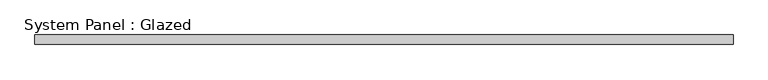
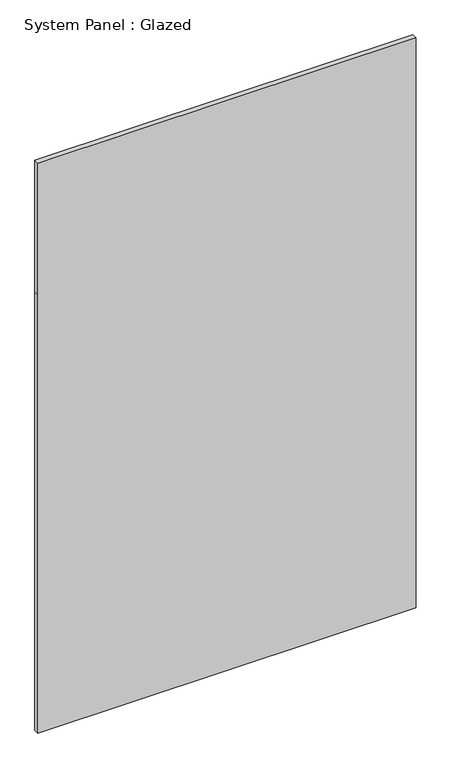
"""IFC4 building model written with IfcOpenShell, lengths in millimetres: plate geometry, System Panel : Glazed."""

import ifcopenshell
import ifcopenshell.guid

model = None  # the IFC model being written
_history = None  # IfcOwnerHistory: only IFC2X3 demands one
_inside = {}  # id of a spatial element -> (the spatial element, [elements in it])
_under = {}  # id of a project, library or spatial element -> (it, [spatial elements below it])
_declared = {}  # id of a project -> (the project, [libraries it declares])
_typed = {}  # id of a type object -> (the type object, [elements of that type])
_made_of = {}  # id of a material, layer set ... -> (it, [elements and type objects made of it])


def new_model(schema):
    """Start an empty IFC model of exactly this schema.

    Asked for "IFC4X3", IfcOpenShell would pick the latest addendum, in which some entities
    have other attributes; the version numbers below select the first issue.
    IFC2X3 requires an IfcOwnerHistory on every rooted entity: one is made here for all.
    """
    global model, _history
    if schema == "IFC4X3":
        model = ifcopenshell.file(schema_version=(4, 3, 0, 0))
    else:
        model = ifcopenshell.file(schema=schema)
    _inside.clear()
    _under.clear()
    _declared.clear()
    _typed.clear()
    _made_of.clear()
    _history = None
    if model.schema == "IFC2X3":
        org = make("IfcOrganization", Name="unknown")
        user = make(
            "IfcPersonAndOrganization",
            ThePerson=make("IfcPerson", FamilyName="unknown"),
            TheOrganization=org,
        )
        app = make(
            "IfcApplication",
            ApplicationDeveloper=org,
            Version="unknown",
            ApplicationFullName="unknown",
            ApplicationIdentifier="unknown",
        )
        _history = make(
            "IfcOwnerHistory",
            OwningUser=user,
            OwningApplication=app,
            ChangeAction="ADDED",
            CreationDate=0,
        )
    return model


def make(cls, **values):
    """One entity of the class cls with the attributes given. An attribute that is None is left unset."""
    return model.create_entity(
        cls, **{name: value for name, value in values.items() if value is not None}
    )


def rooted(cls, **values):
    """An entity with a GlobalId (a new one), such as an element, a storey or a relation."""
    return make(cls, GlobalId=ifcopenshell.guid.new(), OwnerHistory=_history, **values)


def si_unit(unit_type, name, prefix=None):
    """IfcSIUnit, for example si_unit("LENGTHUNIT", "METRE", prefix="MILLI")."""
    return make("IfcSIUnit", UnitType=unit_type, Prefix=prefix, Name=name)


def assignment(units):
    """IfcUnitAssignment: the units of a project."""
    return None if units is None else make("IfcUnitAssignment", Units=units)


def point(xyz):
    """IfcCartesianPoint."""
    return None if xyz is None else make("IfcCartesianPoint", Coordinates=xyz)


def direction(xyz):
    """IfcDirection."""
    return None if xyz is None else make("IfcDirection", DirectionRatios=xyz)


def frame(location, z_axis=None, x_axis=None):
    """IfcAxis2Placement3D, a coordinate frame: its origin and axes. An axis left out is left unset."""
    return make(
        "IfcAxis2Placement3D",
        Location=point(location),
        Axis=direction(z_axis),
        RefDirection=direction(x_axis),
    )


def origin():
    """The frame at (0, 0, 0) with its axes left unset."""
    return frame((0.0, 0.0, 0.0))


def place(relative_to, where):
    """IfcLocalPlacement: puts the frame where relative to a parent placement (None: the world)."""
    return make(
        "IfcLocalPlacement", PlacementRelTo=relative_to, RelativePlacement=where
    )


def context(
    kind, dimensions, precision=None, world=None, true_north=None, identifier=None
):
    """IfcGeometricRepresentationContext, for example the 3D "Model" context."""
    return make(
        "IfcGeometricRepresentationContext",
        ContextIdentifier=identifier,
        ContextType=kind,
        CoordinateSpaceDimension=dimensions,
        Precision=precision,
        WorldCoordinateSystem=world,
        TrueNorth=true_north,
    )


def project(units=None, contexts=None):
    """IfcProject with its units and contexts."""
    return rooted(
        "IfcProject",
        Name="project",
        RepresentationContexts=contexts,
        UnitsInContext=assignment(units),
    )


def spatial(cls, under=None, at=None, **own):
    """A site, building, storey or space (cls), placed at a placement, below another one or the project."""
    s = rooted(cls, ObjectPlacement=at, **own)
    if under is not None:
        _under.setdefault(under.id(), (under, []))[1].append(s)
    return s


def polyline(points):
    """IfcPolyline through the points."""
    return make("IfcPolyline", Points=[point(p) for p in points])


def outline(outer, holes=None, kind="AREA"):
    """IfcArbitraryClosedProfileDef: a profile drawn as a closed curve; with holes, ...WithVoids."""
    if holes is None:
        return make("IfcArbitraryClosedProfileDef", ProfileType=kind, OuterCurve=outer)
    return make(
        "IfcArbitraryProfileDefWithVoids",
        ProfileType=kind,
        OuterCurve=outer,
        InnerCurves=holes,
    )


def extrude(swept, where, along, depth):
    """IfcExtrudedAreaSolid: the profile swept, set in the frame where, extruded along a direction by depth."""
    return make(
        "IfcExtrudedAreaSolid",
        SweptArea=swept,
        Position=where,
        ExtrudedDirection=direction(along),
        Depth=depth,
    )


def shape(context_of_items, identifier, shape_type, items):
    """IfcShapeRepresentation: the items that make up one representation, for example the "Body"."""
    return make(
        "IfcShapeRepresentation",
        ContextOfItems=context_of_items,
        RepresentationIdentifier=identifier,
        RepresentationType=shape_type,
        Items=items,
    )


def source(mapping_origin, context_of_items, identifier, shape_type, items):
    """IfcRepresentationMap: a shape defined once, which mapped items show again and again."""
    return make(
        "IfcRepresentationMap",
        MappingOrigin=mapping_origin,
        MappedRepresentation=shape(context_of_items, identifier, shape_type, items),
    )


def transform(
    local_origin,
    x_axis=None,
    y_axis=None,
    z_axis=None,
    scale=None,
    scale2=None,
    scale3=None,
    uniform=True,
):
    """IfcCartesianTransformationOperator3D, or its non-uniform kind. x_axis, y_axis, z_axis: its Axis1, 2, 3."""
    if uniform:
        return make(
            "IfcCartesianTransformationOperator3D",
            Axis1=direction(x_axis),
            Axis2=direction(y_axis),
            LocalOrigin=point(local_origin),
            Scale=scale,
            Axis3=direction(z_axis),
        )
    return make(
        "IfcCartesianTransformationOperator3DnonUniform",
        Axis1=direction(x_axis),
        Axis2=direction(y_axis),
        LocalOrigin=point(local_origin),
        Scale=scale,
        Axis3=direction(z_axis),
        Scale2=scale2,
        Scale3=scale3,
    )


def mapped(mapping_source, mapping_target):
    """IfcMappedItem: shows the shape of a source again, moved by a transform."""
    return make(
        "IfcMappedItem", MappingSource=mapping_source, MappingTarget=mapping_target
    )


def made_of(thing, what):
    """Note that an element or type object is made of a material, layer set ...; save() writes the relation."""
    if what is not None:
        _made_of.setdefault(what.id(), (what, []))[1].append(thing)
    return thing


def element(
    cls,
    number,
    at=None,
    inside=None,
    cuts=None,
    type_object=None,
    material=None,
    context=None,
    identifier="Body",
    shape_type=None,
    held_by="IfcProductDefinitionShape",
    body=None,
    shapes=None,
    **own,
):
    """One element of the class cls, such as IfcWall. Its Tag is "e" and its number.

    at: its placement. inside: the storey or other place that contains it. cuts: it is an
    opening in that element (IfcRelVoidsElement). A single representation is given by context,
    identifier, shape_type and body (its items); several are given by shapes. held_by: the class
    of the entity that holds the representations. save() writes the other relations.
    """
    e = rooted(cls, Tag="e%d" % number, ObjectPlacement=at, **own)
    if body is not None:
        shapes = [shape(context, identifier, shape_type, body)]
    if shapes is not None:
        e.Representation = make(held_by, Representations=shapes)
    if inside is not None:
        _inside.setdefault(inside.id(), (inside, []))[1].append(e)
    if cuts is not None:
        rooted(
            "IfcRelVoidsElement", RelatingBuildingElement=cuts, RelatedOpeningElement=e
        )
    if type_object is not None:
        _typed.setdefault(type_object.id(), (type_object, []))[1].append(e)
    return made_of(e, material)


def aggregate(whole, parts):
    """IfcRelAggregates: a whole, such as a stair, and the parts it consists of."""
    return rooted("IfcRelAggregates", RelatingObject=whole, RelatedObjects=parts)


def save(model, path):
    """Write the relations noted so far, then the file.

    IfcRelAggregates (storeys below a building ...), IfcRelContainedInSpatialStructure (elements
    in a storey), IfcRelDefinesByType, IfcRelAssociatesMaterial and IfcRelDeclares: one each for
    every whole, place, type object, material and project.
    """
    for whole, parts in _under.values():
        aggregate(whole, parts)
    for where, things in _inside.values():
        rooted(
            "IfcRelContainedInSpatialStructure",
            RelatedElements=things,
            RelatingStructure=where,
        )
    for kind, things in _typed.values():
        rooted("IfcRelDefinesByType", RelatedObjects=things, RelatingType=kind)
    for what, things in _made_of.values():
        rooted("IfcRelAssociatesMaterial", RelatedObjects=things, RelatingMaterial=what)
    for by, libraries in _declared.values():
        rooted("IfcRelDeclares", RelatingContext=by, RelatedDefinitions=libraries)
    model.write(path)


def system_panel_glazed_e39fabdc(model_context):
    return source(origin(), model_context, "Body", "SweptSolid", [
        extrude(outline(polyline([(0.0, -918.0833333), (0.0, 918.0833333), (2250.0, 918.0833333), (2925.0, 918.0833333), (2925.0, -918.0833333), (2250.0, -918.0833333), (0.0, -918.0833333)])), frame((0.0, 24.5, 0.0), z_axis=(0.0, 1.0, 0.0), x_axis=(0.0, 0.0, 1.0)), (0.0, 0.0, 1.0), 25.0),
    ])


if __name__ == "__main__":
    model = new_model("IFC4")
    model_context = context("Model", 3, world=origin())
    ifc_project = project(units=[si_unit("LENGTHUNIT", "METRE", prefix="MILLI")], contexts=[model_context])
    site = spatial("IfcSite", under=ifc_project)
    building = spatial("IfcBuilding", under=site)
    placement = place(None, origin())
    system_panel_glazed_shape = system_panel_glazed_e39fabdc(model_context)
    element("IfcPlate", 1, ObjectType="System Panel : Glazed", at=placement, inside=building, context=model_context, shape_type="MappedRepresentation", body=[
        mapped(system_panel_glazed_shape, transform((0.0, 0.0, 0.0), x_axis=(1.0, 0.0, 0.0), y_axis=(0.0, 1.0, 0.0), z_axis=(0.0, 0.0, 1.0))),
    ])
    save(model, "model.ifc")

# Revit data of these elements
# Element 1 (IfcPlate, "System Panel : Glazed")
#   Materials on its faces: "Glass"
# Materials
#   "Glass": class "Glass", colour RGB 0 128 192, transparency 0.9
